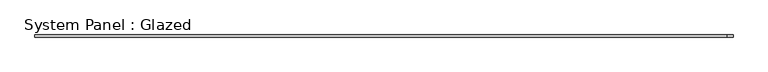
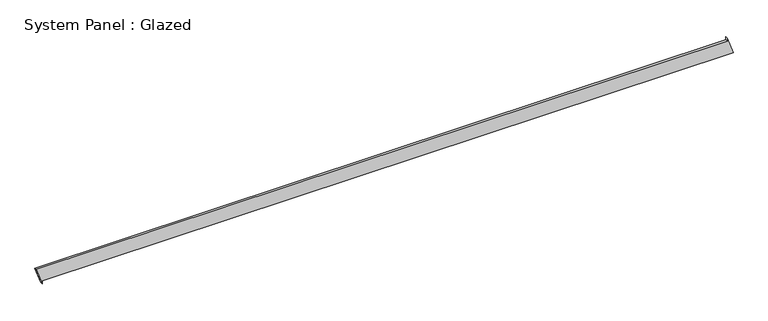
"""IFC4 building model written with IfcOpenShell, lengths in millimetres: plate geometry, System Panel : Glazed."""

import ifcopenshell
import ifcopenshell.guid

model = None  # the IFC model being written
_history = None  # IfcOwnerHistory: only IFC2X3 demands one
_inside = {}  # id of a spatial element -> (the spatial element, [elements in it])
_under = {}  # id of a project, library or spatial element -> (it, [spatial elements below it])
_declared = {}  # id of a project -> (the project, [libraries it declares])
_typed = {}  # id of a type object -> (the type object, [elements of that type])
_made_of = {}  # id of a material, layer set ... -> (it, [elements and type objects made of it])


def new_model(schema):
    """Start an empty IFC model of exactly this schema.

    Asked for "IFC4X3", IfcOpenShell would pick the latest addendum, in which some entities
    have other attributes; the version numbers below select the first issue.
    IFC2X3 requires an IfcOwnerHistory on every rooted entity: one is made here for all.
    """
    global model, _history
    if schema == "IFC4X3":
        model = ifcopenshell.file(schema_version=(4, 3, 0, 0))
    else:
        model = ifcopenshell.file(schema=schema)
    _inside.clear()
    _under.clear()
    _declared.clear()
    _typed.clear()
    _made_of.clear()
    _history = None
    if model.schema == "IFC2X3":
        org = make("IfcOrganization", Name="unknown")
        user = make(
            "IfcPersonAndOrganization",
            ThePerson=make("IfcPerson", FamilyName="unknown"),
            TheOrganization=org,
        )
        app = make(
            "IfcApplication",
            ApplicationDeveloper=org,
            Version="unknown",
            ApplicationFullName="unknown",
            ApplicationIdentifier="unknown",
        )
        _history = make(
            "IfcOwnerHistory",
            OwningUser=user,
            OwningApplication=app,
            ChangeAction="ADDED",
            CreationDate=0,
        )
    return model


def make(cls, **values):
    """One entity of the class cls with the attributes given. An attribute that is None is left unset."""
    return model.create_entity(
        cls, **{name: value for name, value in values.items() if value is not None}
    )


def rooted(cls, **values):
    """An entity with a GlobalId (a new one), such as an element, a storey or a relation."""
    return make(cls, GlobalId=ifcopenshell.guid.new(), OwnerHistory=_history, **values)


def si_unit(unit_type, name, prefix=None):
    """IfcSIUnit, for example si_unit("LENGTHUNIT", "METRE", prefix="MILLI")."""
    return make("IfcSIUnit", UnitType=unit_type, Prefix=prefix, Name=name)


def assignment(units):
    """IfcUnitAssignment: the units of a project."""
    return None if units is None else make("IfcUnitAssignment", Units=units)


def point(xyz):
    """IfcCartesianPoint."""
    return None if xyz is None else make("IfcCartesianPoint", Coordinates=xyz)


def direction(xyz):
    """IfcDirection."""
    return None if xyz is None else make("IfcDirection", DirectionRatios=xyz)


def frame(location, z_axis=None, x_axis=None):
    """IfcAxis2Placement3D, a coordinate frame: its origin and axes. An axis left out is left unset."""
    return make(
        "IfcAxis2Placement3D",
        Location=point(location),
        Axis=direction(z_axis),
        RefDirection=direction(x_axis),
    )


def origin():
    """The frame at (0, 0, 0) with its axes left unset."""
    return frame((0.0, 0.0, 0.0))


def place(relative_to, where):
    """IfcLocalPlacement: puts the frame where relative to a parent placement (None: the world)."""
    return make(
        "IfcLocalPlacement", PlacementRelTo=relative_to, RelativePlacement=where
    )


def context(
    kind, dimensions, precision=None, world=None, true_north=None, identifier=None
):
    """IfcGeometricRepresentationContext, for example the 3D "Model" context."""
    return make(
        "IfcGeometricRepresentationContext",
        ContextIdentifier=identifier,
        ContextType=kind,
        CoordinateSpaceDimension=dimensions,
        Precision=precision,
        WorldCoordinateSystem=world,
        TrueNorth=true_north,
    )


def project(units=None, contexts=None):
    """IfcProject with its units and contexts."""
    return rooted(
        "IfcProject",
        Name="project",
        RepresentationContexts=contexts,
        UnitsInContext=assignment(units),
    )


def spatial(cls, under=None, at=None, **own):
    """A site, building, storey or space (cls), placed at a placement, below another one or the project."""
    s = rooted(cls, ObjectPlacement=at, **own)
    if under is not None:
        _under.setdefault(under.id(), (under, []))[1].append(s)
    return s


def polyline(points):
    """IfcPolyline through the points."""
    return make("IfcPolyline", Points=[point(p) for p in points])


def outline(outer, holes=None, kind="AREA"):
    """IfcArbitraryClosedProfileDef: a profile drawn as a closed curve; with holes, ...WithVoids."""
    if holes is None:
        return make("IfcArbitraryClosedProfileDef", ProfileType=kind, OuterCurve=outer)
    return make(
        "IfcArbitraryProfileDefWithVoids",
        ProfileType=kind,
        OuterCurve=outer,
        InnerCurves=holes,
    )


def extrude(swept, where, along, depth):
    """IfcExtrudedAreaSolid: the profile swept, set in the frame where, extruded along a direction by depth."""
    return make(
        "IfcExtrudedAreaSolid",
        SweptArea=swept,
        Position=where,
        ExtrudedDirection=direction(along),
        Depth=depth,
    )


def shape(context_of_items, identifier, shape_type, items):
    """IfcShapeRepresentation: the items that make up one representation, for example the "Body"."""
    return make(
        "IfcShapeRepresentation",
        ContextOfItems=context_of_items,
        RepresentationIdentifier=identifier,
        RepresentationType=shape_type,
        Items=items,
    )


def source(mapping_origin, context_of_items, identifier, shape_type, items):
    """IfcRepresentationMap: a shape defined once, which mapped items show again and again."""
    return make(
        "IfcRepresentationMap",
        MappingOrigin=mapping_origin,
        MappedRepresentation=shape(context_of_items, identifier, shape_type, items),
    )


def transform(
    local_origin,
    x_axis=None,
    y_axis=None,
    z_axis=None,
    scale=None,
    scale2=None,
    scale3=None,
    uniform=True,
):
    """IfcCartesianTransformationOperator3D, or its non-uniform kind. x_axis, y_axis, z_axis: its Axis1, 2, 3."""
    if uniform:
        return make(
            "IfcCartesianTransformationOperator3D",
            Axis1=direction(x_axis),
            Axis2=direction(y_axis),
            LocalOrigin=point(local_origin),
            Scale=scale,
            Axis3=direction(z_axis),
        )
    return make(
        "IfcCartesianTransformationOperator3DnonUniform",
        Axis1=direction(x_axis),
        Axis2=direction(y_axis),
        LocalOrigin=point(local_origin),
        Scale=scale,
        Axis3=direction(z_axis),
        Scale2=scale2,
        Scale3=scale3,
    )


def mapped(mapping_source, mapping_target):
    """IfcMappedItem: shows the shape of a source again, moved by a transform."""
    return make(
        "IfcMappedItem", MappingSource=mapping_source, MappingTarget=mapping_target
    )


def made_of(thing, what):
    """Note that an element or type object is made of a material, layer set ...; save() writes the relation."""
    if what is not None:
        _made_of.setdefault(what.id(), (what, []))[1].append(thing)
    return thing


def element(
    cls,
    number,
    at=None,
    inside=None,
    cuts=None,
    type_object=None,
    material=None,
    context=None,
    identifier="Body",
    shape_type=None,
    held_by="IfcProductDefinitionShape",
    body=None,
    shapes=None,
    **own,
):
    """One element of the class cls, such as IfcWall. Its Tag is "e" and its number.

    at: its placement. inside: the storey or other place that contains it. cuts: it is an
    opening in that element (IfcRelVoidsElement). A single representation is given by context,
    identifier, shape_type and body (its items); several are given by shapes. held_by: the class
    of the entity that holds the representations. save() writes the other relations.
    """
    e = rooted(cls, Tag="e%d" % number, ObjectPlacement=at, **own)
    if body is not None:
        shapes = [shape(context, identifier, shape_type, body)]
    if shapes is not None:
        e.Representation = make(held_by, Representations=shapes)
    if inside is not None:
        _inside.setdefault(inside.id(), (inside, []))[1].append(e)
    if cuts is not None:
        rooted(
            "IfcRelVoidsElement", RelatingBuildingElement=cuts, RelatedOpeningElement=e
        )
    if type_object is not None:
        _typed.setdefault(type_object.id(), (type_object, []))[1].append(e)
    return made_of(e, material)


def aggregate(whole, parts):
    """IfcRelAggregates: a whole, such as a stair, and the parts it consists of."""
    return rooted("IfcRelAggregates", RelatingObject=whole, RelatedObjects=parts)


def save(model, path):
    """Write the relations noted so far, then the file.

    IfcRelAggregates (storeys below a building ...), IfcRelContainedInSpatialStructure (elements
    in a storey), IfcRelDefinesByType, IfcRelAssociatesMaterial and IfcRelDeclares: one each for
    every whole, place, type object, material and project.
    """
    for whole, parts in _under.values():
        aggregate(whole, parts)
    for where, things in _inside.values():
        rooted(
            "IfcRelContainedInSpatialStructure",
            RelatedElements=things,
            RelatingStructure=where,
        )
    for kind, things in _typed.values():
        rooted("IfcRelDefinesByType", RelatedObjects=things, RelatingType=kind)
    for what, things in _made_of.values():
        rooted("IfcRelAssociatesMaterial", RelatedObjects=things, RelatingMaterial=what)
    for by, libraries in _declared.values():
        rooted("IfcRelDeclares", RelatingContext=by, RelatedDefinitions=libraries)
    model.write(path)


def system_panel_glazed_a3f05b8f(model_context):
    return source(origin(), model_context, "Body", "SweptSolid", [
        extrude(outline(polyline([(0.0, -3958.100606), (35.3553391, -3958.100606), (35.3553391, 4027.4732247), (235.6210783, 3958.4712631), (200.2657393, 3958.4719436), (200.1120339, -4027.4732247), (0.0, -3958.100606)])), frame((0.0, -49.5, 0.0), z_axis=(0.0, 1.0, 0.0), x_axis=(0.0, 0.0, 1.0)), (0.0, 0.0, 1.0), 25.0),
    ])


if __name__ == "__main__":
    model = new_model("IFC4")
    model_context = context("Model", 3, world=origin())
    ifc_project = project(units=[si_unit("LENGTHUNIT", "METRE", prefix="MILLI")], contexts=[model_context])
    site = spatial("IfcSite", under=ifc_project)
    building = spatial("IfcBuilding", under=site)
    placement = place(None, origin())
    system_panel_glazed_shape = system_panel_glazed_a3f05b8f(model_context)
    element("IfcPlate", 1, ObjectType="System Panel : Glazed", at=placement, inside=building, context=model_context, shape_type="MappedRepresentation", body=[
        mapped(system_panel_glazed_shape, transform((0.0, 0.0, 0.0), x_axis=(1.0, 0.0, 0.0), y_axis=(0.0, 1.0, 0.0), z_axis=(0.0, 0.0, 1.0))),
    ])
    save(model, "model.ifc")

# Revit data of these elements
# Element 1 (IfcPlate, "System Panel : Glazed")
#   Materials on its faces: "Glass"
# Materials
#   "Glass": class "Glass", colour RGB 218 227 224, transparency 0.85, Description = "Soda Lime Glass", Cost = 0
